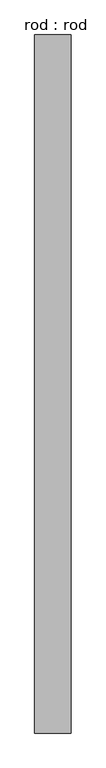
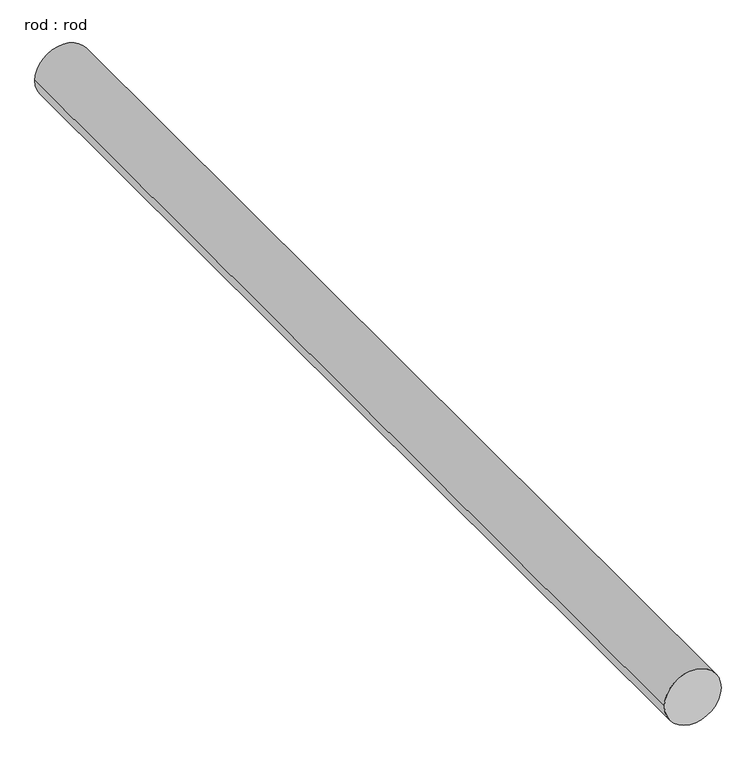
"""IFC4 building model written with IfcOpenShell, lengths in millimetres: proxy geometry, rod : rod."""

from ifc_helpers import new_model, si_unit, point, frame, frame_2d, origin, place, context, project, spatial, circle_curve, trimmed, segment, composite_curve, outline, extrude, source, transform, mapped, element, save


def rod_rod_d7f3904c(model_context):
    return source(origin(), model_context, "Body", "SweptSolid", [
        extrude(outline(composite_curve([segment(trimmed(circle_curve(frame_2d((0.0108462, 0.0)), 200.0), [point((0.0108462, 200.0))], [point((0.0108462, -200.0))], False, "CARTESIAN"), True, "CONTINUOUS"), segment(trimmed(circle_curve(frame_2d((0.0108462, 0.0)), 200.0), [point((0.0108462, -200.0))], [point((0.0108462, 200.0))], False, "CARTESIAN"), True, "CONTINUOUS")], self_intersect=False)), frame((0.0, 240.7118952, 0.0), z_axis=(0.0, 1.0, 0.0), x_axis=(0.0, 0.0, 1.0)), (0.0, 0.0, 1.0), 7704.0334403),
    ])


if __name__ == "__main__":
    model = new_model("IFC4")
    model_context = context("Model", 3, world=origin())
    ifc_project = project(units=[si_unit("LENGTHUNIT", "METRE", prefix="MILLI")], contexts=[model_context])
    site = spatial("IfcSite", under=ifc_project)
    building = spatial("IfcBuilding", under=site)
    placement = place(None, origin())
    rod_rod_shape = rod_rod_d7f3904c(model_context)
    element("IfcBuildingElementProxy", 1, Name="rod : rod", ObjectType="rod : rod", at=placement, inside=building, context=model_context, shape_type="MappedRepresentation", body=[
        mapped(rod_rod_shape, transform((0.0, 0.0, 0.0), x_axis=(1.0, 0.0, 0.0), y_axis=(0.0, 1.0, 0.0), z_axis=(0.0, 0.0, 1.0))),
    ])
    save(model, "model.ifc")

# Revit data of these elements
# Type "rod : rod"
#   Default Elevation = 0
